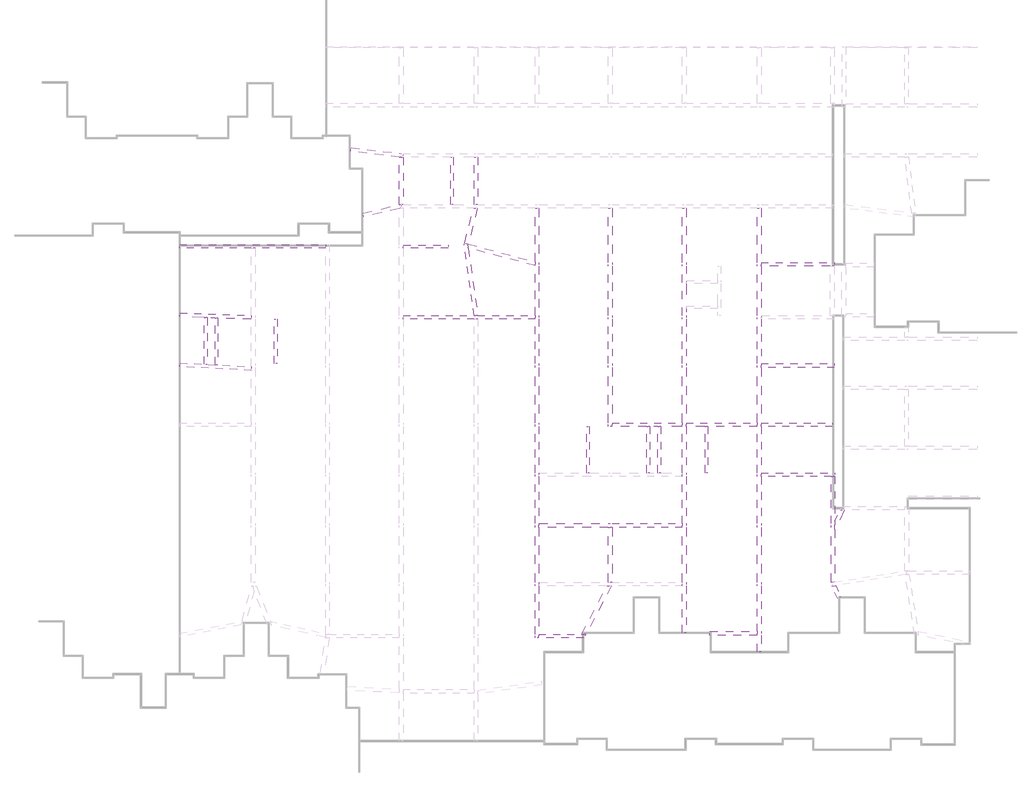
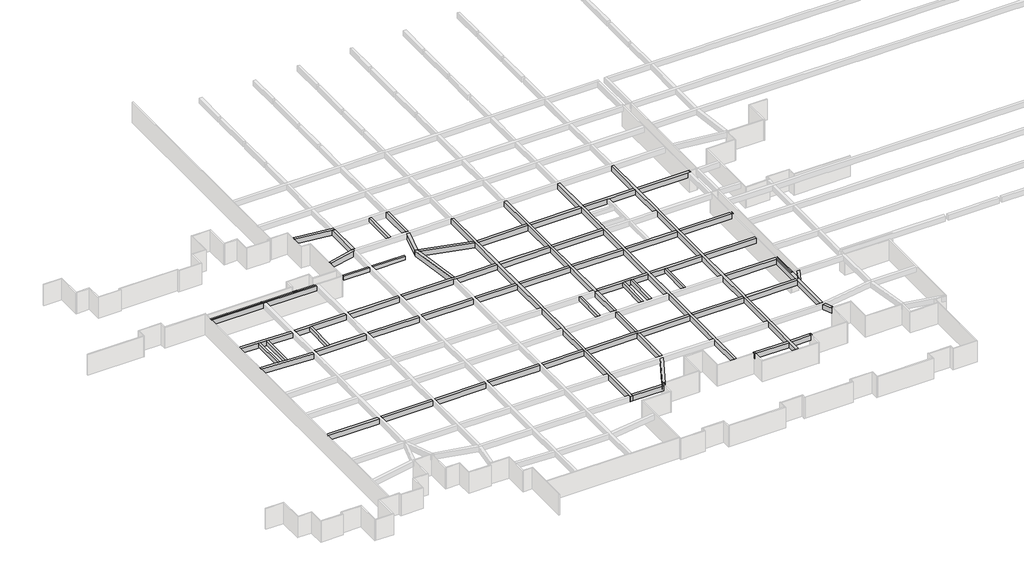
# One storey, part 10 of 16: 38 beams.
"""IFC4 building model written with IfcOpenShell, lengths in millimetres."""

from ifc_helpers import new_model, si_unit, frame, origin, place, context, project, spatial, polyline, outline, extrude, faceted_brep, element, save

model = new_model("IFC4")

# Units and contexts
model_context = context("Model", 3, world=origin())
ifc_project = project(units=[si_unit("LENGTHUNIT", "METRE", prefix="MILLI")], contexts=[model_context])

# Site, building, storey
site = spatial("IfcSite", under=ifc_project)
building = spatial("IfcBuilding", under=site)
storey = spatial("IfcBuildingStorey", under=building, Name="户型图", Elevation=0.0)

# Beams
placement = place(None, origin())
element("IfcBeam", 1, ObjectType="混凝土 - 矩形梁 : KL_beam", at=placement, inside=storey, context=model_context, shape_type="Brep", body=[
    faceted_brep([(202886.3957871, -166173.8814198, 3300.0), (202886.3957871, -166173.8814198, 2500.0), (202837.6480497, -166570.8998804, 2500.0), (202837.6480497, -166570.8998804, 3300.0), (208472.2780151, -167262.7454466, 3300.0), (208474.7427196, -167242.6720388, 3300.0), (208521.0257524, -166865.7269859, 3300.0), (208121.0257524, -166816.6131615, 3300.0), (208121.0257524, -167219.6170917, 3300.0), (208308.7932284, -167242.6720388, 3300.0), (208472.2780151, -167262.7454466, 2500.0), (208121.0257524, -167219.6170917, 2500.0), (208308.7932284, -167242.6720388, 2500.0), (208521.0257524, -166865.7269859, 2500.0), (208474.7427196, -167242.6720388, 2500.0), (208121.0257524, -166816.6131615, 2500.0)], [[[0, 1, 2, 3]], [[4, 5, 6, 7, 0, 3, 8, 9]], [[10, 4, 9, 8, 3, 2, 11, 12]], [[13, 14, 10, 12, 11, 2, 1, 15]], [[6, 13, 15, 1, 0, 7]], [[6, 5, 4, 10, 14, 13]]]),
])
element("IfcBeam", 2, ObjectType="混凝土 - 矩形梁 : KL_beam", at=placement, inside=storey, context=model_context, shape_type="Brep", body=[
    faceted_brep([(204160.2720993, -173284.8120655, 3300.0), (204160.2720993, -173284.8120655, 2500.0), (204250.2525211, -173674.5600915, 2500.0), (204250.2525211, -173674.5600915, 3300.0), (208320.403704, -172734.8916503, 3300.0), (208274.8294606, -172334.8916503, 3300.0), (208121.0257524, -172370.4000342, 3300.0), (208121.0257524, -172780.9216773, 3300.0), (208320.403704, -172734.8916503, 2500.0), (208121.0257524, -172780.9216773, 2500.0), (208274.8294606, -172334.8916503, 2500.0), (208121.0257524, -172370.4000342, 2500.0)], [[[0, 1, 2, 3]], [[4, 5, 6, 0, 3, 7]], [[8, 4, 7, 3, 2, 9]], [[10, 8, 9, 2, 1, 11]], [[5, 10, 11, 1, 0, 6]], [[5, 4, 8, 10]]]),
])
element("IfcBeam", 3, ObjectType="混凝土 - 矩形梁 : KL_beam", at=placement, inside=storey, context=model_context, shape_type="SweptSolid", body=[
    extrude(outline(polyline([(208308.7932284, -167242.6720388), (208472.2780151, -167262.7454466), (208474.7427196, -167242.6720388), (208521.0257524, -167242.6720388), (208521.0257524, -172334.8916503), (208274.8294606, -172334.8916503), (208121.0257524, -172370.4000342), (208121.0257524, -167242.6720388), (208308.7932284, -167242.6720388)])), frame((0.0, 0.0, 2500.0), z_axis=(0.0, 0.0, 1.0), x_axis=(1.0, 0.0, 0.0)), (0.0, 0.0, 1.0), 800.0),
])
element("IfcBeam", 4, ObjectType="混凝土 - 矩形梁 : KL_beam", at=placement, inside=storey, context=model_context, shape_type="SweptSolid", body=[
    extrude(outline(polyline([(216198.8904026, -167242.6720388), (216598.8904026, -167242.6720388), (216598.8904026, -172334.8916503), (216198.8904026, -172334.8916503), (216198.8904026, -167242.6720388)])), frame((0.0, 0.0, 2500.0), z_axis=(0.0, 0.0, 1.0), x_axis=(1.0, 0.0, 0.0)), (0.0, 0.0, 1.0), 800.0),
])
element("IfcBeam", 5, ObjectType="混凝土 - 矩形梁 : KL_beam", at=placement, inside=storey, context=model_context, shape_type="Brep", body=[
    faceted_brep([(215177.5544053, -176523.2702865, 3300.0), (215117.8929954, -176757.7149155, 3300.0), (216187.0478754, -184365.1471774, 3300.0), (216590.9789045, -184365.1471774, 3300.0), (215561.5342494, -177040.2678478, 3300.0), (215524.9612283, -176780.0372808, 3300.0), (215501.0573924, -176609.9526507, 3300.0), (216590.9789045, -184365.1471774, 2500.0), (215561.5342494, -177040.2678478, 2500.0), (215524.9612283, -176780.0372808, 2500.0), (215501.0573924, -176609.9526507, 2500.0), (215117.8929954, -176757.7149155, 2500.0), (215177.5544053, -176523.2702865, 2500.0), (216187.0478754, -184365.1471774, 2500.0)], [[[0, 1, 2, 3, 4, 5, 6]], [[6, 5, 4, 3, 7, 8, 9, 10]], [[11, 12, 10, 9, 8, 7, 13]], [[1, 11, 13, 2]], [[1, 0, 12, 11]], [[2, 13, 7, 3]], [[12, 0, 6, 10]]]),
])
element("IfcBeam", 6, ObjectType="混凝土 - 矩形梁 : KL_beam", at=placement, inside=storey, context=model_context, shape_type="Brep", body=[
    faceted_brep([(215501.0573924, -176609.9526507, 3300.0), (215524.9612283, -176780.0372808, 3300.0), (215563.9554515, -176626.8061348, 3300.0), (216554.3688646, -172734.8916503, 3300.0), (216141.6200419, -172734.8916503, 3300.0), (215177.5544053, -176523.2702865, 3300.0), (215524.9612283, -176780.0372808, 2500.0), (215563.9554515, -176626.8061348, 2500.0), (216554.3688646, -172734.8916503, 2500.0), (215501.0573924, -176609.9526507, 2500.0), (215177.5544053, -176523.2702865, 2500.0), (216141.6200419, -172734.8916503, 2500.0)], [[[0, 1, 2, 3, 4, 5]], [[1, 6, 7, 8, 3, 2]], [[6, 9, 10, 11, 8, 7]], [[10, 5, 4, 11]], [[1, 0, 9, 6]], [[4, 3, 8, 11]], [[9, 0, 5, 10]]]),
])
element("IfcBeam", 7, ObjectType="混凝土 - 矩形梁 : KL_beam", at=placement, inside=storey, context=model_context, shape_type="Brep", body=[
    faceted_brep([(222798.8904026, -219234.8916503, 3300.0), (223198.8904026, -219234.8916503, 3300.0), (223198.8904026, -218834.8916503, 3300.0), (223198.8904026, -213630.8034485, 3300.0), (223198.8904026, -213230.8034485, 3300.0), (223198.8904026, -207265.1471774, 3300.0), (223198.8904026, -206865.1471774, 3300.0), (223198.8904026, -201765.1471774, 3300.0), (223198.8904026, -201365.1471774, 3300.0), (223198.8904026, -196365.1471774, 3300.0), (223198.8904026, -195965.1471774, 3300.0), (223198.8904026, -189965.1471774, 3300.0), (223198.8904026, -189565.1471774, 3300.0), (223198.8904026, -184765.1471774, 3300.0), (223198.8904026, -184365.1471774, 3300.0), (223198.8904026, -179026.0461868, 3300.0), (223198.8904026, -178626.0461868, 3300.0), (223198.8904026, -172734.8916503, 3300.0), (222798.8904026, -172734.8916503, 3300.0), (222798.8904026, -178565.4011123, 3300.0), (222798.8904026, -178979.5115844, 3300.0), (222798.8904026, -184365.1471774, 3300.0), (222798.8904026, -184765.1471774, 3300.0), (222798.8904026, -189565.1471774, 3300.0), (222798.8904026, -189965.1471774, 3300.0), (222798.8904026, -195965.1471774, 3300.0), (222798.8904026, -196365.1471774, 3300.0), (222798.8904026, -201365.1471774, 3300.0), (222798.8904026, -201765.1471774, 3300.0), (222798.8904026, -206865.1471774, 3300.0), (222798.8904026, -207265.1471774, 3300.0), (222798.8904026, -213230.8034485, 3300.0), (222798.8904026, -213630.8034485, 3300.0), (222798.8904026, -218834.8916503, 3300.0), (222798.8904026, -219234.8916503, 2500.0), (222798.8904026, -172734.8916503, 2500.0), (222798.8904026, -178565.4011123, 2500.0), (222798.8904026, -178979.5115844, 2500.0), (222798.8904026, -184365.1471774, 2500.0), (222798.8904026, -184765.1471774, 2500.0), (222798.8904026, -189565.1471774, 2500.0), (222798.8904026, -189965.1471774, 2500.0), (222798.8904026, -195965.1471774, 2500.0), (222798.8904026, -196365.1471774, 2500.0), (222798.8904026, -201365.1471774, 2500.0), (222798.8904026, -201765.1471774, 2500.0), (222798.8904026, -206865.1471774, 2500.0), (222798.8904026, -207265.1471774, 2500.0), (222798.8904026, -213230.8034485, 2500.0), (222798.8904026, -213630.8034485, 2500.0), (222798.8904026, -218834.8916503, 2500.0), (223198.8904026, -219234.8916503, 2500.0), (223198.8904026, -172734.8916503, 2500.0), (223198.8904026, -178626.0461868, 2500.0), (223198.8904026, -179026.0461868, 2500.0), (223198.8904026, -184365.1471774, 2500.0), (223198.8904026, -184765.1471774, 2500.0), (223198.8904026, -189565.1471774, 2500.0), (223198.8904026, -189965.1471774, 2500.0), (223198.8904026, -195965.1471774, 2500.0), (223198.8904026, -196365.1471774, 2500.0), (223198.8904026, -201365.1471774, 2500.0), (223198.8904026, -201765.1471774, 2500.0), (223198.8904026, -206865.1471774, 2500.0), (223198.8904026, -207265.1471774, 2500.0), (223198.8904026, -213230.8034485, 2500.0), (223198.8904026, -213630.8034485, 2500.0), (223198.8904026, -218834.8916503, 2500.0)], [[[0, 1, 2, 3, 4, 5, 6, 7, 8, 9, 10, 11, 12, 13, 14, 15, 16, 17, 18, 19, 20, 21, 22, 23, 24, 25, 26, 27, 28, 29, 30, 31, 32, 33]], [[34, 0, 33, 32, 31, 30, 29, 28, 27, 26, 25, 24, 23, 22, 21, 20, 19, 18, 35, 36, 37, 38, 39, 40, 41, 42, 43, 44, 45, 46, 47, 48, 49, 50]], [[51, 34, 50, 49, 48, 47, 46, 45, 44, 43, 42, 41, 40, 39, 38, 37, 36, 35, 52, 53, 54, 55, 56, 57, 58, 59, 60, 61, 62, 63, 64, 65, 66, 67]], [[1, 51, 67, 66, 65, 64, 63, 62, 61, 60, 59, 58, 57, 56, 55, 54, 53, 52, 17, 16, 15, 14, 13, 12, 11, 10, 9, 8, 7, 6, 5, 4, 3, 2]], [[18, 17, 52, 35]], [[1, 0, 34, 51]]]),
])
element("IfcBeam", 8, ObjectType="混凝土 - 矩形梁 : KL_beam", at=placement, inside=storey, context=model_context, shape_type="Brep", body=[
    faceted_brep([(228058.8638251, -219234.8916503, 3300.0), (228271.5475977, -218834.8916503, 3300.0), (227818.5195775, -218834.8916503, 3300.0), (223198.8904026, -218834.8916503, 3300.0), (223198.8904026, -219234.8916503, 3300.0), (228058.8638251, -219234.8916503, 2500.0), (223198.8904026, -219234.8916503, 2500.0), (228271.5475977, -218834.8916503, 2500.0), (223198.8904026, -218834.8916503, 2500.0), (227818.5195775, -218834.8916503, 2500.0)], [[[0, 1, 2, 3, 4]], [[5, 0, 4, 6]], [[7, 5, 6, 8, 9]], [[1, 7, 9, 8, 3, 2]], [[4, 3, 8, 6]], [[1, 0, 5, 7]]]),
])
element("IfcBeam", 9, ObjectType="混凝土 - 矩形梁 : KL_beam", at=placement, inside=storey, context=model_context, shape_type="Brep", body=[
    faceted_brep([(230718.438254, -196365.1471774, 3300.0), (231118.438254, -196365.1471774, 3300.0), (231118.438254, -195965.1471774, 3300.0), (231118.438254, -189965.1471774, 3300.0), (231118.438254, -189565.1471774, 3300.0), (231118.438254, -184765.1471774, 3300.0), (231118.438254, -184365.1471774, 3300.0), (231118.438254, -179026.0461868, 3300.0), (231118.438254, -178626.0461868, 3300.0), (231118.438254, -172734.8916503, 3300.0), (230718.438254, -172734.8916503, 3300.0), (230718.438254, -178626.0461868, 3300.0), (230718.438254, -179026.0461868, 3300.0), (230718.438254, -184365.1471774, 3300.0), (230718.438254, -184765.1471774, 3300.0), (230718.438254, -189565.1471774, 3300.0), (230718.438254, -189965.1471774, 3300.0), (230718.438254, -195965.1471774, 3300.0), (230718.438254, -196365.1471774, 2500.0), (230718.438254, -172734.8916503, 2500.0), (230718.438254, -178626.0461868, 2500.0), (230718.438254, -179026.0461868, 2500.0), (230718.438254, -184365.1471774, 2500.0), (230718.438254, -184765.1471774, 2500.0), (230718.438254, -189565.1471774, 2500.0), (230718.438254, -189965.1471774, 2500.0), (230718.438254, -195965.1471774, 2500.0), (231118.438254, -196365.1471774, 2500.0), (231118.438254, -172734.8916503, 2500.0), (231118.438254, -178626.0461868, 2500.0), (231118.438254, -179026.0461868, 2500.0), (231118.438254, -184365.1471774, 2500.0), (231118.438254, -184765.1471774, 2500.0), (231118.438254, -189565.1471774, 2500.0), (231118.438254, -189965.1471774, 2500.0), (231118.438254, -195965.1471774, 2500.0)], [[[0, 1, 2, 3, 4, 5, 6, 7, 8, 9, 10, 11, 12, 13, 14, 15, 16, 17]], [[18, 0, 17, 16, 15, 14, 13, 12, 11, 10, 19, 20, 21, 22, 23, 24, 25, 26]], [[27, 18, 26, 25, 24, 23, 22, 21, 20, 19, 28, 29, 30, 31, 32, 33, 34, 35]], [[1, 27, 35, 34, 33, 32, 31, 30, 29, 28, 9, 8, 7, 6, 5, 4, 3, 2]], [[10, 9, 28, 19]], [[1, 0, 18, 27]]]),
])
element("IfcBeam", 10, ObjectType="混凝土 - 矩形梁 : KL_beam", at=placement, inside=storey, context=model_context, shape_type="Brep", body=[
    faceted_brep([(239118.438254, -218673.2637363, 3300.0), (238718.438254, -218673.2637363, 3300.0), (238718.438254, -218673.2637363, 2500.0), (239118.438254, -218673.2637363, 2500.0), (239118.438254, -213630.8034485, 3300.0), (239118.438254, -213230.8034485, 3300.0), (239118.438254, -207265.1471774, 3300.0), (239118.438254, -206865.1471774, 3300.0), (239118.438254, -201765.1471774, 3300.0), (239118.438254, -201365.1471774, 3300.0), (239118.438254, -196365.1471774, 3300.0), (239118.438254, -195965.1471774, 3300.0), (239118.438254, -189965.1471774, 3300.0), (239118.438254, -189565.1471774, 3300.0), (239118.438254, -184765.1471774, 3300.0), (239118.438254, -184365.1471774, 3300.0), (239118.438254, -183615.1471774, 3300.0), (239118.438254, -183315.1471774, 3300.0), (239118.438254, -180876.0461868, 3300.0), (239118.438254, -180576.0461868, 3300.0), (239118.438254, -179026.0461868, 3300.0), (239118.438254, -178626.0461868, 3300.0), (239118.438254, -172734.8916503, 3300.0), (238718.438254, -172734.8916503, 3300.0), (238718.438254, -178626.0461868, 3300.0), (238718.438254, -179026.0461868, 3300.0), (238718.438254, -184365.1471774, 3300.0), (238718.438254, -184765.1471774, 3300.0), (238718.438254, -189565.1471774, 3300.0), (238718.438254, -189965.1471774, 3300.0), (238718.438254, -195965.1471774, 3300.0), (238718.438254, -196365.1471774, 3300.0), (238718.438254, -201365.1471774, 3300.0), (238718.438254, -201765.1471774, 3300.0), (238718.438254, -206865.1471774, 3300.0), (238718.438254, -207265.1471774, 3300.0), (238718.438254, -213230.8034485, 3300.0), (238718.438254, -213630.8034485, 3300.0), (238718.438254, -172734.8916503, 2500.0), (238718.438254, -178626.0461868, 2500.0), (238718.438254, -179026.0461868, 2500.0), (238718.438254, -184365.1471774, 2500.0), (238718.438254, -184765.1471774, 2500.0), (238718.438254, -189565.1471774, 2500.0), (238718.438254, -189965.1471774, 2500.0), (238718.438254, -195965.1471774, 2500.0), (238718.438254, -196365.1471774, 2500.0), (238718.438254, -201365.1471774, 2500.0), (238718.438254, -201765.1471774, 2500.0), (238718.438254, -206865.1471774, 2500.0), (238718.438254, -207265.1471774, 2500.0), (238718.438254, -213230.8034485, 2500.0), (238718.438254, -213630.8034485, 2500.0), (239118.438254, -172734.8916503, 2500.0), (239118.438254, -178626.0461868, 2500.0), (239118.438254, -179026.0461868, 2500.0), (239118.438254, -184365.1471774, 2500.0), (239118.438254, -184765.1471774, 2500.0), (239118.438254, -189565.1471774, 2500.0), (239118.438254, -189965.1471774, 2500.0), (239118.438254, -195965.1471774, 2500.0), (239118.438254, -196365.1471774, 2500.0), (239118.438254, -201365.1471774, 2500.0), (239118.438254, -201765.1471774, 2500.0), (239118.438254, -206865.1471774, 2500.0), (239118.438254, -207265.1471774, 2500.0), (239118.438254, -213230.8034485, 2500.0), (239118.438254, -213630.8034485, 2500.0)], [[[0, 1, 2, 3]], [[1, 0, 4, 5, 6, 7, 8, 9, 10, 11, 12, 13, 14, 15, 16, 17, 18, 19, 20, 21, 22, 23, 24, 25, 26, 27, 28, 29, 30, 31, 32, 33, 34, 35, 36, 37]], [[2, 1, 37, 36, 35, 34, 33, 32, 31, 30, 29, 28, 27, 26, 25, 24, 23, 38, 39, 40, 41, 42, 43, 44, 45, 46, 47, 48, 49, 50, 51, 52]], [[3, 2, 52, 51, 50, 49, 48, 47, 46, 45, 44, 43, 42, 41, 40, 39, 38, 53, 54, 55, 56, 57, 58, 59, 60, 61, 62, 63, 64, 65, 66, 67]], [[0, 3, 67, 66, 65, 64, 63, 62, 61, 60, 59, 58, 57, 56, 55, 54, 53, 22, 21, 20, 19, 18, 17, 16, 15, 14, 13, 12, 11, 10, 9, 8, 7, 6, 5, 4]], [[23, 22, 53, 38]]]),
])
element("IfcBeam", 11, ObjectType="混凝土 - 矩形梁 : KL_beam", at=placement, inside=storey, context=model_context, shape_type="Brep", body=[
    faceted_brep([(247218.438254, -220773.3230967, 3300.0), (246818.438254, -220773.3230967, 3300.0), (246818.438254, -220773.3230967, 2500.0), (247218.438254, -220773.3230967, 2500.0), (247218.438254, -218948.6524453, 3300.0), (247218.438254, -218548.6524453, 3300.0), (247218.438254, -213630.8034485, 3300.0), (247218.438254, -213230.8034485, 3300.0), (247218.438254, -207265.1471774, 3300.0), (247218.438254, -206865.1471774, 3300.0), (247218.438254, -201765.1471774, 3300.0), (247218.438254, -201365.1471774, 3300.0), (247218.438254, -196365.1471774, 3300.0), (247218.438254, -195965.1471774, 3300.0), (247218.438254, -189965.1471774, 3300.0), (247218.438254, -189565.1471774, 3300.0), (247218.438254, -184765.1471774, 3300.0), (247218.438254, -184365.1471774, 3300.0), (247218.438254, -179026.0461868, 3300.0), (247218.438254, -178626.0461868, 3300.0), (247218.438254, -172734.8916503, 3300.0), (246818.438254, -172734.8916503, 3300.0), (246818.438254, -178626.0461868, 3300.0), (246818.438254, -179026.0461868, 3300.0), (246818.438254, -184365.1471774, 3300.0), (246818.438254, -184765.1471774, 3300.0), (246818.438254, -189565.1471774, 3300.0), (246818.438254, -189965.1471774, 3300.0), (246818.438254, -195965.1471774, 3300.0), (246818.438254, -196365.1471774, 3300.0), (246818.438254, -201365.1471774, 3300.0), (246818.438254, -201765.1471774, 3300.0), (246818.438254, -206865.1471774, 3300.0), (246818.438254, -207265.1471774, 3300.0), (246818.438254, -213230.8034485, 3300.0), (246818.438254, -213630.8034485, 3300.0), (246818.438254, -218548.6524453, 3300.0), (246818.438254, -218948.6524453, 3300.0), (246818.438254, -172734.8916503, 2500.0), (246818.438254, -178626.0461868, 2500.0), (246818.438254, -179026.0461868, 2500.0), (246818.438254, -184365.1471774, 2500.0), (246818.438254, -184765.1471774, 2500.0), (246818.438254, -189565.1471774, 2500.0), (246818.438254, -189965.1471774, 2500.0), (246818.438254, -195965.1471774, 2500.0), (246818.438254, -196365.1471774, 2500.0), (246818.438254, -201365.1471774, 2500.0), (246818.438254, -201765.1471774, 2500.0), (246818.438254, -206865.1471774, 2500.0), (246818.438254, -207265.1471774, 2500.0), (246818.438254, -213230.8034485, 2500.0), (246818.438254, -213630.8034485, 2500.0), (246818.438254, -218548.6524453, 2500.0), (246818.438254, -218948.6524453, 2500.0), (247218.438254, -172734.8916503, 2500.0), (247218.438254, -178626.0461868, 2500.0), (247218.438254, -179026.0461868, 2500.0), (247218.438254, -184365.1471774, 2500.0), (247218.438254, -184765.1471774, 2500.0), (247218.438254, -189565.1471774, 2500.0), (247218.438254, -189965.1471774, 2500.0), (247218.438254, -195965.1471774, 2500.0), (247218.438254, -196365.1471774, 2500.0), (247218.438254, -201365.1471774, 2500.0), (247218.438254, -201765.1471774, 2500.0), (247218.438254, -206865.1471774, 2500.0), (247218.438254, -207265.1471774, 2500.0), (247218.438254, -213230.8034485, 2500.0), (247218.438254, -213630.8034485, 2500.0), (247218.438254, -218548.6524453, 2500.0), (247218.438254, -218948.6524453, 2500.0)], [[[0, 1, 2, 3]], [[1, 0, 4, 5, 6, 7, 8, 9, 10, 11, 12, 13, 14, 15, 16, 17, 18, 19, 20, 21, 22, 23, 24, 25, 26, 27, 28, 29, 30, 31, 32, 33, 34, 35, 36, 37]], [[2, 1, 37, 36, 35, 34, 33, 32, 31, 30, 29, 28, 27, 26, 25, 24, 23, 22, 21, 38, 39, 40, 41, 42, 43, 44, 45, 46, 47, 48, 49, 50, 51, 52, 53, 54]], [[3, 2, 54, 53, 52, 51, 50, 49, 48, 47, 46, 45, 44, 43, 42, 41, 40, 39, 38, 55, 56, 57, 58, 59, 60, 61, 62, 63, 64, 65, 66, 67, 68, 69, 70, 71]], [[0, 3, 71, 70, 69, 68, 67, 66, 65, 64, 63, 62, 61, 60, 59, 58, 57, 56, 55, 20, 19, 18, 17, 16, 15, 14, 13, 12, 11, 10, 9, 8, 7, 6, 5, 4]], [[21, 20, 55, 38]]]),
])
element("IfcBeam", 12, ObjectType="混凝土 - 矩形梁 : KL_beam", at=placement, inside=storey, context=model_context, shape_type="Brep", body=[
    faceted_brep([(192508.6297316, -184365.1471774, 3300.0), (192508.6297316, -184765.1471774, 3300.0), (194594.1756261, -184765.1471774, 3300.0), (194894.1756261, -184765.1471774, 3300.0), (200145.9052003, -184765.1471774, 3300.0), (200145.9052003, -184365.1471774, 3300.0), (192508.6297316, -184765.1471774, 2500.0), (200145.9052003, -184765.1471774, 2500.0), (192508.6297316, -184365.1471774, 2500.0), (200145.9052003, -184365.1471774, 2500.0)], [[[0, 1, 2, 3, 4, 5]], [[1, 6, 7, 4, 3, 2]], [[6, 8, 9, 7]], [[8, 0, 5, 9]], [[1, 0, 8, 6]], [[5, 4, 7, 9]]]),
    faceted_brep([(238718.438254, -184365.1471774, 3300.0), (238718.438254, -184765.1471774, 3300.0), (238718.438254, -184765.1471774, 2500.0), (238718.438254, -184365.1471774, 2500.0), (231118.438254, -184765.1471774, 3300.0), (231118.438254, -184365.1471774, 3300.0), (231118.438254, -184365.1471774, 2500.0), (231118.438254, -184765.1471774, 2500.0)], [[[0, 1, 2, 3]], [[4, 5, 6, 7]], [[1, 0, 5, 4]], [[2, 1, 4, 7]], [[3, 2, 7, 6]], [[0, 3, 6, 5]]]),
    faceted_brep([(208121.0257524, -184365.1471774, 3300.0), (208121.0257524, -184765.1471774, 3300.0), (208121.0257524, -184765.1471774, 2500.0), (208121.0257524, -184365.1471774, 2500.0), (200545.9052003, -184765.1471774, 3300.0), (200545.9052003, -184365.1471774, 3300.0), (200545.9052003, -184365.1471774, 2500.0), (200545.9052003, -184765.1471774, 2500.0)], [[[0, 1, 2, 3]], [[4, 5, 6, 7]], [[1, 0, 5, 4]], [[2, 1, 4, 7]], [[3, 2, 7, 6]], [[0, 3, 6, 5]]]),
    faceted_brep([(208521.0257524, -184765.1471774, 3300.0), (208521.0257524, -184365.1471774, 3300.0), (208521.0257524, -184365.1471774, 2500.0), (208521.0257524, -184765.1471774, 2500.0), (222798.8904026, -184365.1471774, 3300.0), (222798.8904026, -184765.1471774, 3300.0), (222798.8904026, -184765.1471774, 2500.0), (222798.8904026, -184365.1471774, 2500.0), (216206.9772993, -184765.1471774, 3300.0), (216606.9772993, -184765.1471774, 3300.0), (216590.9789045, -184365.1471774, 3300.0), (216187.0478754, -184365.1471774, 3300.0), (216206.9772993, -184765.1471774, 2500.0), (216606.9772993, -184765.1471774, 2500.0), (216187.0478754, -184365.1471774, 2500.0), (216590.9789045, -184365.1471774, 2500.0)], [[[0, 1, 2, 3]], [[4, 5, 6, 7]], [[1, 0, 8, 9, 5, 4, 10, 11]], [[0, 3, 12, 13, 6, 5, 9, 8]], [[3, 2, 14, 15, 7, 6, 13, 12]], [[2, 1, 11, 10, 4, 7, 15, 14]]]),
    faceted_brep([(223198.8904026, -184365.1471774, 3300.0), (223198.8904026, -184765.1471774, 3300.0), (230718.438254, -184765.1471774, 3300.0), (230718.438254, -184365.1471774, 3300.0), (223198.8904026, -184765.1471774, 2500.0), (230718.438254, -184765.1471774, 2500.0), (223198.8904026, -184365.1471774, 2500.0), (230718.438254, -184365.1471774, 2500.0)], [[[0, 1, 2, 3]], [[1, 4, 5, 2]], [[4, 6, 7, 5]], [[6, 0, 3, 7]], [[1, 0, 6, 4]], [[3, 2, 5, 7]]]),
])
element("IfcBeam", 13, ObjectType="混凝土 - 矩形梁 : KL_beam", at=placement, inside=storey, context=model_context, shape_type="SweptSolid", body=[
    extrude(outline(polyline([(215561.5342494, -177040.2678478), (215524.9612283, -176780.0372808), (215563.9554515, -176626.8061348), (222798.8904026, -178565.4011123), (222798.8904026, -178979.5115844), (215561.5342494, -177040.2678478)])), frame((0.0, 0.0, 2500.0), z_axis=(0.0, 0.0, 1.0), x_axis=(1.0, 0.0, 0.0)), (0.0, 0.0, 1.0), 800.0),
])
element("IfcBeam", 14, ObjectType="混凝土 - 矩形梁 : KL_beam", at=placement, inside=storey, context=model_context, shape_type="Brep", body=[
    faceted_brep([(223198.8904026, -178626.0461868, 3300.0), (223198.8904026, -179026.0461868, 3300.0), (230718.438254, -179026.0461868, 3300.0), (230718.438254, -178626.0461868, 3300.0), (223198.8904026, -179026.0461868, 2500.0), (230718.438254, -179026.0461868, 2500.0), (223198.8904026, -178626.0461868, 2500.0), (230718.438254, -178626.0461868, 2500.0)], [[[0, 1, 2, 3]], [[1, 4, 5, 2]], [[4, 6, 7, 5]], [[6, 0, 3, 7]], [[1, 0, 6, 4]], [[3, 2, 5, 7]]]),
    faceted_brep([(231118.438254, -179026.0461868, 3300.0), (231118.438254, -178626.0461868, 3300.0), (231118.438254, -178626.0461868, 2500.0), (231118.438254, -179026.0461868, 2500.0), (238718.438254, -178626.0461868, 3300.0), (238718.438254, -179026.0461868, 3300.0), (238718.438254, -179026.0461868, 2500.0), (238718.438254, -178626.0461868, 2500.0)], [[[0, 1, 2, 3]], [[4, 5, 6, 7]], [[1, 0, 5, 4]], [[0, 3, 6, 5]], [[3, 2, 7, 6]], [[2, 1, 4, 7]]]),
    faceted_brep([(239118.438254, -178626.0461868, 3300.0), (239118.438254, -179026.0461868, 3300.0), (242568.438254, -179026.0461868, 3300.0), (242868.438254, -179026.0461868, 3300.0), (246818.438254, -179026.0461868, 3300.0), (246818.438254, -178626.0461868, 3300.0), (239118.438254, -179026.0461868, 2500.0), (246818.438254, -179026.0461868, 2500.0), (239118.438254, -178626.0461868, 2500.0), (246818.438254, -178626.0461868, 2500.0)], [[[0, 1, 2, 3, 4, 5]], [[1, 6, 7, 4, 3, 2]], [[6, 8, 9, 7]], [[8, 0, 5, 9]], [[1, 0, 8, 6]], [[5, 4, 7, 9]]]),
    faceted_brep([(247218.438254, -179026.0461868, 3300.0), (247218.438254, -178626.0461868, 3300.0), (247218.438254, -178626.0461868, 2500.0), (247218.438254, -179026.0461868, 2500.0), (255118.438254, -178626.0461868, 3300.0), (255118.438254, -179026.0461868, 3300.0), (255118.438254, -179026.0461868, 2500.0), (255118.438254, -178626.0461868, 2500.0), (254718.438254, -179026.0461868, 3300.0), (254718.438254, -179026.0461868, 2500.0)], [[[0, 1, 2, 3]], [[4, 5, 6, 7]], [[5, 4, 1, 0, 8]], [[6, 5, 8, 0, 3, 9]], [[7, 6, 9, 3, 2]], [[4, 7, 2, 1]]]),
])
element("IfcBeam", 15, ObjectType="混凝土 - 矩形梁 : KL_beam", at=placement, inside=storey, context=model_context, shape_type="Brep", body=[
    faceted_brep([(184345.9052003, -177080.869332, 3300.0), (184345.9052003, -176680.869332, 3300.0), (184345.9052003, -176680.869332, 2500.0), (184345.9052003, -177080.869332, 2500.0), (192108.6297316, -177080.869332, 3300.0), (192508.6297316, -177080.869332, 3300.0), (200145.9052003, -177080.869332, 3300.0), (200145.9052003, -176680.869332, 3300.0), (200145.9052003, -176680.869332, 2500.0), (200145.9052003, -177080.869332, 2500.0), (192508.6297316, -177080.869332, 2500.0), (192108.6297316, -177080.869332, 2500.0)], [[[0, 1, 2, 3]], [[1, 0, 4, 5, 6, 7]], [[2, 1, 7, 8]], [[3, 2, 8, 9, 10, 11]], [[0, 3, 11, 10, 9, 6, 5, 4]], [[7, 6, 9, 8]]]),
])
element("IfcBeam", 16, ObjectType="混凝土 - 矩形梁 : KL_beam", at=placement, inside=storey, context=model_context, shape_type="Brep", body=[
    faceted_brep([(184367.3625426, -184487.9539253, 3300.0), (184381.3223413, -184088.1975945, 3300.0), (184381.3223413, -184088.1975945, 2500.0), (184367.3625426, -184487.9539253, 2500.0), (187022.6367576, -184580.6781441, 3300.0), (187322.6367576, -184591.154375, 3300.0), (188191.4243298, -184621.4931055, 3300.0), (188491.4243298, -184631.9693364, 3300.0), (192108.6297316, -184758.2849324, 3300.0), (192108.6297316, -184358.0411147, 3300.0), (192108.6297316, -184358.0411147, 2500.0), (192108.6297316, -184758.2849324, 2500.0)], [[[0, 1, 2, 3]], [[1, 0, 4, 5, 6, 7, 8, 9]], [[2, 1, 9, 10]], [[3, 2, 10, 11]], [[0, 3, 11, 8, 7, 6, 5, 4]], [[9, 8, 11, 10]]]),
])
element("IfcBeam", 17, ObjectType="混凝土 - 矩形梁 : KL_beam", at=placement, inside=storey, context=model_context, shape_type="Brep", body=[
    faceted_brep([(184363.9013118, -189889.0560732, 3300.0), (184384.8356943, -189489.6042592, 3300.0), (184384.8356943, -189489.6042592, 2500.0), (184363.9013118, -189889.0560732, 2500.0), (192108.6297316, -190294.9400908, 3300.0), (192108.6297316, -189894.3911524, 3300.0), (188491.4243298, -189704.8214501, 3300.0), (188191.4243298, -189689.0991163, 3300.0), (187322.6367576, -189643.567889, 3300.0), (187022.6367576, -189627.8455552, 3300.0), (192108.6297316, -189894.3911524, 2500.0), (192108.6297316, -190294.9400908, 2500.0)], [[[0, 1, 2, 3]], [[1, 0, 4, 5, 6, 7, 8, 9]], [[2, 1, 9, 8, 7, 6, 5, 10]], [[3, 2, 10, 11]], [[0, 3, 11, 4]], [[5, 4, 11, 10]]]),
])
element("IfcBeam", 18, ObjectType="混凝土 - 矩形梁 : KL_beam", at=placement, inside=storey, context=model_context, shape_type="Brep", body=[
    faceted_brep([(231118.438254, -195965.1471774, 3300.0), (231118.438254, -196365.1471774, 3300.0), (234868.438254, -196365.1471774, 3300.0), (235168.438254, -196365.1471774, 3300.0), (236068.438254, -196365.1471774, 3300.0), (236368.438254, -196365.1471774, 3300.0), (238718.438254, -196365.1471774, 3300.0), (238718.438254, -195965.1471774, 3300.0), (231118.438254, -196365.1471774, 2500.0), (238718.438254, -196365.1471774, 2500.0), (231118.438254, -195965.1471774, 2500.0), (238718.438254, -195965.1471774, 2500.0)], [[[0, 1, 2, 3, 4, 5, 6, 7]], [[1, 8, 9, 6, 5, 4, 3, 2]], [[8, 10, 11, 9]], [[10, 0, 7, 11]], [[1, 0, 10, 8]], [[7, 6, 9, 11]]]),
])
element("IfcBeam", 19, ObjectType="混凝土 - 矩形梁 : KL_beam", at=placement, inside=storey, context=model_context, shape_type="Brep", body=[
    faceted_brep([(239118.438254, -195965.1471774, 3300.0), (239118.438254, -196365.1471774, 3300.0), (241168.438254, -196365.1471774, 3300.0), (241468.438254, -196365.1471774, 3300.0), (246818.438254, -196365.1471774, 3300.0), (246818.438254, -195965.1471774, 3300.0), (239118.438254, -196365.1471774, 2500.0), (246818.438254, -196365.1471774, 2500.0), (239118.438254, -195965.1471774, 2500.0), (246818.438254, -195965.1471774, 2500.0)], [[[0, 1, 2, 3, 4, 5]], [[1, 6, 7, 4, 3, 2]], [[6, 8, 9, 7]], [[8, 0, 5, 9]], [[1, 0, 8, 6]], [[5, 4, 7, 9]]]),
])
element("IfcBeam", 20, ObjectType="混凝土 - 矩形梁 : KL_beam", at=placement, inside=storey, context=model_context, shape_type="Brep", body=[
    faceted_brep([(255153.6937038, -189565.1471774, 3300.0), (255153.6937038, -189965.1471774, 3300.0), (255153.6937038, -189965.1471774, 2500.0), (255153.6937038, -189565.1471774, 2500.0), (247218.438254, -189565.1471774, 3300.0), (247218.438254, -189965.1471774, 3300.0), (247218.438254, -189965.1471774, 2500.0), (247218.438254, -189565.1471774, 2500.0)], [[[0, 1, 2, 3]], [[1, 0, 4, 5]], [[2, 1, 5, 6]], [[3, 2, 6, 7]], [[0, 3, 7, 4]], [[5, 4, 7, 6]]]),
    faceted_brep([(192508.6297316, -189965.1471774, 3300.0), (192508.6297316, -189565.1471774, 3300.0), (192508.6297316, -189565.1471774, 2500.0), (192508.6297316, -189965.1471774, 2500.0), (200145.9052003, -189565.1471774, 3300.0), (200145.9052003, -189965.1471774, 3300.0), (200145.9052003, -189965.1471774, 2500.0), (200145.9052003, -189565.1471774, 2500.0), (194894.1756261, -189565.1471774, 3300.0), (194594.1756261, -189565.1471774, 3300.0)], [[[0, 1, 2, 3]], [[4, 5, 6, 7]], [[1, 0, 5, 4, 8, 9]], [[0, 3, 6, 5]], [[3, 2, 7, 6]], [[2, 1, 9, 8, 4, 7]]]),
    faceted_brep([(208121.0257524, -189565.1471774, 3300.0), (208121.0257524, -189965.1471774, 3300.0), (208121.0257524, -189965.1471774, 2500.0), (208121.0257524, -189565.1471774, 2500.0), (200545.9052003, -189565.1471774, 3300.0), (200545.9052003, -189965.1471774, 3300.0), (200545.9052003, -189965.1471774, 2500.0), (200545.9052003, -189565.1471774, 2500.0)], [[[0, 1, 2, 3]], [[1, 0, 4, 5]], [[2, 1, 5, 6]], [[3, 2, 6, 7]], [[0, 3, 7, 4]], [[5, 4, 7, 6]]]),
    faceted_brep([(208521.0257524, -189965.1471774, 3300.0), (208521.0257524, -189565.1471774, 3300.0), (208521.0257524, -189565.1471774, 2500.0), (208521.0257524, -189965.1471774, 2500.0), (216206.9772993, -189565.1471774, 3300.0), (216206.9772993, -189965.1471774, 3300.0), (216206.9772993, -189965.1471774, 2500.0), (216206.9772993, -189565.1471774, 2500.0)], [[[0, 1, 2, 3]], [[4, 5, 6, 7]], [[1, 0, 5, 4]], [[0, 3, 6, 5]], [[3, 2, 7, 6]], [[2, 1, 4, 7]]]),
    faceted_brep([(216606.9772993, -189965.1471774, 3300.0), (216606.9772993, -189565.1471774, 3300.0), (216606.9772993, -189565.1471774, 2500.0), (216606.9772993, -189965.1471774, 2500.0), (222798.8904026, -189565.1471774, 3300.0), (222798.8904026, -189965.1471774, 3300.0), (222798.8904026, -189965.1471774, 2500.0), (222798.8904026, -189565.1471774, 2500.0)], [[[0, 1, 2, 3]], [[4, 5, 6, 7]], [[1, 0, 5, 4]], [[0, 3, 6, 5]], [[3, 2, 7, 6]], [[2, 1, 4, 7]]]),
    faceted_brep([(223198.8904026, -189965.1471774, 3300.0), (223198.8904026, -189565.1471774, 3300.0), (223198.8904026, -189565.1471774, 2500.0), (223198.8904026, -189965.1471774, 2500.0), (230718.438254, -189565.1471774, 3300.0), (230718.438254, -189965.1471774, 3300.0), (230718.438254, -189965.1471774, 2500.0), (230718.438254, -189565.1471774, 2500.0)], [[[0, 1, 2, 3]], [[4, 5, 6, 7]], [[1, 0, 5, 4]], [[0, 3, 6, 5]], [[3, 2, 7, 6]], [[2, 1, 4, 7]]]),
    faceted_brep([(231118.438254, -189965.1471774, 3300.0), (231118.438254, -189565.1471774, 3300.0), (231118.438254, -189565.1471774, 2500.0), (231118.438254, -189965.1471774, 2500.0), (238718.438254, -189565.1471774, 3300.0), (238718.438254, -189965.1471774, 3300.0), (238718.438254, -189965.1471774, 2500.0), (238718.438254, -189565.1471774, 2500.0)], [[[0, 1, 2, 3]], [[4, 5, 6, 7]], [[1, 0, 5, 4]], [[0, 3, 6, 5]], [[3, 2, 7, 6]], [[2, 1, 4, 7]]]),
    faceted_brep([(239118.438254, -189965.1471774, 3300.0), (239118.438254, -189565.1471774, 3300.0), (239118.438254, -189565.1471774, 2500.0), (239118.438254, -189965.1471774, 2500.0), (246818.438254, -189565.1471774, 3300.0), (246818.438254, -189965.1471774, 3300.0), (246818.438254, -189965.1471774, 2500.0), (246818.438254, -189565.1471774, 2500.0), (242868.438254, -189565.1471774, 3300.0), (242568.438254, -189565.1471774, 3300.0)], [[[0, 1, 2, 3]], [[4, 5, 6, 7]], [[1, 0, 5, 4, 8, 9]], [[0, 3, 6, 5]], [[3, 2, 7, 6]], [[2, 1, 9, 8, 4, 7]]]),
])
element("IfcBeam", 21, ObjectType="混凝土 - 矩形梁 : KL_beam", at=placement, inside=storey, context=model_context, shape_type="Brep", body=[
    faceted_brep([(184374.3285911, -206865.1471774, 3300.0), (184374.3285911, -206865.1471774, 2500.0), (184374.3285911, -207265.1471774, 2500.0), (184374.3285911, -207265.1471774, 3300.0), (192108.6297316, -206865.1471774, 3300.0), (192108.6297316, -207265.1471774, 3300.0), (192108.6297316, -207265.1471774, 2500.0), (192108.6297316, -206865.1471774, 2500.0)], [[[0, 1, 2, 3]], [[4, 5, 6, 7]], [[0, 3, 5, 4]], [[3, 2, 6, 5]], [[2, 1, 7, 6]], [[1, 0, 4, 7]]]),
    faceted_brep([(208521.0257524, -206865.1471774, 3300.0), (208521.0257524, -207265.1471774, 3300.0), (216206.9772993, -207265.1471774, 3300.0), (216206.9772993, -206865.1471774, 3300.0), (208521.0257524, -207265.1471774, 2500.0), (216206.9772993, -207265.1471774, 2500.0), (208521.0257524, -206865.1471774, 2500.0), (216206.9772993, -206865.1471774, 2500.0)], [[[0, 1, 2, 3]], [[1, 4, 5, 2]], [[4, 6, 7, 5]], [[6, 0, 3, 7]], [[1, 0, 6, 4]], [[3, 2, 5, 7]]]),
    faceted_brep([(208121.0257524, -206865.1471774, 3300.0), (208121.0257524, -207265.1471774, 3300.0), (208121.0257524, -207265.1471774, 2500.0), (208121.0257524, -206865.1471774, 2500.0), (200545.9052003, -206865.1471774, 3300.0), (200545.9052003, -207265.1471774, 3300.0), (200545.9052003, -207265.1471774, 2500.0), (200545.9052003, -206865.1471774, 2500.0)], [[[0, 1, 2, 3]], [[1, 0, 4, 5]], [[2, 1, 5, 6]], [[3, 2, 6, 7]], [[0, 3, 7, 4]], [[5, 4, 7, 6]]]),
    faceted_brep([(216606.9772993, -207265.1471774, 3300.0), (216606.9772993, -206865.1471774, 3300.0), (216606.9772993, -206865.1471774, 2500.0), (216606.9772993, -207265.1471774, 2500.0), (222798.8904026, -206865.1471774, 3300.0), (222798.8904026, -207265.1471774, 3300.0), (222798.8904026, -207265.1471774, 2500.0), (222798.8904026, -206865.1471774, 2500.0)], [[[0, 1, 2, 3]], [[4, 5, 6, 7]], [[1, 0, 5, 4]], [[0, 3, 6, 5]], [[3, 2, 7, 6]], [[2, 1, 4, 7]]]),
    faceted_brep([(223198.8904026, -206865.1471774, 3300.0), (223198.8904026, -207265.1471774, 3300.0), (230718.438254, -207265.1471774, 3300.0), (231118.438254, -207265.1471774, 3300.0), (238718.438254, -207265.1471774, 3300.0), (238718.438254, -206865.1471774, 3300.0), (231118.438254, -206865.1471774, 3300.0), (230718.438254, -206865.1471774, 3300.0), (223198.8904026, -207265.1471774, 2500.0), (230718.438254, -207265.1471774, 2500.0), (231118.438254, -207265.1471774, 2500.0), (238718.438254, -207265.1471774, 2500.0), (223198.8904026, -206865.1471774, 2500.0), (230718.438254, -206865.1471774, 2500.0), (231118.438254, -206865.1471774, 2500.0), (238718.438254, -206865.1471774, 2500.0)], [[[0, 1, 2, 3, 4, 5, 6, 7]], [[1, 8, 9, 10, 11, 4, 3, 2]], [[8, 12, 13, 14, 15, 11, 10, 9]], [[12, 0, 7, 6, 5, 15, 14, 13]], [[1, 0, 12, 8]], [[5, 4, 11, 15]]]),
    faceted_brep([(239118.438254, -207265.1471774, 3300.0), (239118.438254, -206865.1471774, 3300.0), (239118.438254, -206865.1471774, 2500.0), (239118.438254, -207265.1471774, 2500.0), (246818.438254, -206865.1471774, 3300.0), (246818.438254, -207265.1471774, 3300.0), (246818.438254, -207265.1471774, 2500.0), (246818.438254, -206865.1471774, 2500.0)], [[[0, 1, 2, 3]], [[4, 5, 6, 7]], [[1, 0, 5, 4]], [[0, 3, 6, 5]], [[3, 2, 7, 6]], [[2, 1, 4, 7]]]),
    faceted_brep([(247218.438254, -207265.1471774, 3300.0), (247218.438254, -206865.1471774, 3300.0), (247218.438254, -206865.1471774, 2500.0), (247218.438254, -207265.1471774, 2500.0), (254818.438254, -207265.1471774, 3300.0), (254818.438254, -206865.1471774, 3300.0), (254818.438254, -207265.1471774, 2500.0), (254818.438254, -206865.1471774, 2500.0)], [[[0, 1, 2, 3]], [[1, 0, 4, 5]], [[0, 3, 6, 4]], [[3, 2, 7, 6]], [[2, 1, 5, 7]], [[5, 4, 6, 7]]]),
    faceted_brep([(200145.9052003, -206865.1471774, 3300.0), (200145.9052003, -207265.1471774, 3300.0), (200145.9052003, -207265.1471774, 2500.0), (200145.9052003, -206865.1471774, 2500.0), (192508.6297316, -206865.1471774, 3300.0), (192508.6297316, -207265.1471774, 3300.0), (192508.6297316, -207265.1471774, 2500.0), (192508.6297316, -206865.1471774, 2500.0)], [[[0, 1, 2, 3]], [[1, 0, 4, 5]], [[2, 1, 5, 6]], [[3, 2, 6, 7]], [[0, 3, 7, 4]], [[5, 4, 7, 6]]]),
])
element("IfcBeam", 22, ObjectType="混凝土 - 矩形梁 : KL_beam", at=placement, inside=storey, context=model_context, shape_type="SweptSolid", body=[
    extrude(outline(polyline([(230718.438254, -196365.1471774), (231118.438254, -196365.1471774), (231118.438254, -201365.1471774), (230718.438254, -201365.1471774), (230718.438254, -196365.1471774)])), frame((0.0, 0.0, 2500.0), z_axis=(0.0, 0.0, 1.0), x_axis=(1.0, 0.0, 0.0)), (0.0, 0.0, 1.0), 800.0),
    extrude(outline(polyline([(231118.438254, -213230.8034485), (230718.438254, -213230.8034485), (230718.438254, -207265.1471774), (231118.438254, -207265.1471774), (231118.438254, -213230.8034485)])), frame((0.0, 0.0, 2500.0), z_axis=(0.0, 0.0, 1.0), x_axis=(1.0, 0.0, 0.0)), (0.0, 0.0, 1.0), 800.0),
    extrude(outline(polyline([(230718.438254, -201765.1471774), (231118.438254, -201765.1471774), (231118.438254, -206865.1471774), (230718.438254, -206865.1471774), (230718.438254, -201765.1471774)])), frame((0.0, 0.0, 2500.0), z_axis=(0.0, 0.0, 1.0), x_axis=(1.0, 0.0, 0.0)), (0.0, 0.0, 1.0), 800.0),
])
element("IfcBeam", 23, ObjectType="混凝土 - 矩形梁 : KL_beam", at=placement, inside=storey, context=model_context, shape_type="SweptSolid", body=[
    extrude(outline(polyline([(228271.5475977, -218834.8916503), (227818.5195775, -218834.8916503), (230585.5823575, -213630.8034485), (231038.6103778, -213630.8034485), (228271.5475977, -218834.8916503)])), frame((0.0, 0.0, 2500.0), z_axis=(0.0, 0.0, 1.0), x_axis=(1.0, 0.0, 0.0)), (0.0, 0.0, 1.0), 800.0),
])
element("IfcBeam", 24, ObjectType="混凝土 - 矩形梁 : KL_beam", at=placement, inside=storey, context=model_context, shape_type="Brep", body=[
    faceted_brep([(255218.438254, -201765.1471774, 3300.0), (255218.438254, -201365.1471774, 3300.0), (247218.438254, -201365.1471774, 3300.0), (247218.438254, -201765.1471774, 3300.0), (254818.438254, -201765.1471774, 3300.0), (255218.438254, -201765.1471774, 2500.0), (247218.438254, -201765.1471774, 2500.0), (254818.438254, -201765.1471774, 2500.0), (255218.438254, -201365.1471774, 2500.0), (247218.438254, -201365.1471774, 2500.0)], [[[0, 1, 2, 3, 4]], [[5, 0, 4, 3, 6, 7]], [[8, 5, 7, 6, 9]], [[1, 8, 9, 2]], [[3, 2, 9, 6]], [[1, 0, 5, 8]]]),
])
element("IfcBeam", 25, ObjectType="混凝土 - 矩形梁 : KL_beam", at=placement, inside=storey, context=model_context, shape_type="SweptSolid", body=[
    extrude(outline(polyline([(254918.438254, -195965.1471774), (254918.438254, -196365.1471774), (247218.438254, -196365.1471774), (247218.438254, -195965.1471774), (254918.438254, -195965.1471774)])), frame((0.0, 0.0, 2500.0), z_axis=(0.0, 0.0, 1.0), x_axis=(1.0, 0.0, 0.0)), (0.0, 0.0, 1.0), 800.0),
])
element("IfcBeam", 26, ObjectType="混凝土 - 矩形梁 : KL_beam", at=placement, inside=storey, context=model_context, shape_type="SweptSolid", body=[
    extrude(outline(polyline([(255797.2234219, -205405.1471774), (256242.9655049, -205405.1471774), (255218.438254, -207488.7098397), (255218.438254, -206582.2121741), (255797.2234219, -205405.1471774)])), frame((0.0, 0.0, 2500.0), z_axis=(0.0, 0.0, 1.0), x_axis=(1.0, 0.0, 0.0)), (0.0, 0.0, 1.0), 800.0),
])
element("IfcBeam", 27, ObjectType="混凝土 - 矩形梁 : KL_beam", at=placement, inside=storey, context=model_context, shape_type="Brep", body=[
    faceted_brep([(255218.438254, -201765.1471774, 3300.0), (254818.438254, -201765.1471774, 3300.0), (254818.438254, -206865.1471774, 3300.0), (254818.438254, -207265.1471774, 3300.0), (254818.438254, -213230.8034485, 3300.0), (254958.4785867, -213230.8034485, 3300.0), (255218.438254, -213189.6298821, 3300.0), (255218.438254, -207488.7098397, 3300.0), (255218.438254, -206582.2121741, 3300.0), (254818.438254, -201765.1471774, 2500.0), (254818.438254, -206865.1471774, 2500.0), (254818.438254, -207265.1471774, 2500.0), (254818.438254, -213230.8034485, 2500.0), (255218.438254, -201765.1471774, 2500.0), (255218.438254, -206582.2121741, 2500.0), (255218.438254, -207488.7098397, 2500.0), (255218.438254, -213189.6298821, 2500.0), (254958.4785867, -213230.8034485, 2500.0)], [[[0, 1, 2, 3, 4, 5, 6, 7, 8]], [[1, 9, 10, 11, 12, 4, 3, 2]], [[9, 13, 14, 15, 16, 17, 12, 11, 10]], [[13, 0, 8, 7, 6, 16, 15, 14]], [[1, 0, 13, 9]], [[6, 5, 17, 16]], [[5, 4, 12, 17]]]),
])
element("IfcBeam", 28, ObjectType="混凝土 - 矩形梁 : KL_beam", at=placement, inside=storey, context=model_context, shape_type="SweptSolid", body=[
    extrude(outline(polyline([(250269.2509223, -218548.6524453), (250269.2509223, -218948.6524453), (247218.438254, -218948.6524453), (247218.438254, -218548.6524453), (250269.2509223, -218548.6524453)])), frame((0.0, 0.0, 2500.0), z_axis=(0.0, 0.0, 1.0), x_axis=(1.0, 0.0, 0.0)), (0.0, 0.0, 1.0), 800.0),
    extrude(outline(polyline([(241669.2509223, -218948.6524453), (241669.2509223, -218548.6524453), (246818.438254, -218548.6524453), (246818.438254, -218948.6524453), (241669.2509223, -218948.6524453)])), frame((0.0, 0.0, 2500.0), z_axis=(0.0, 0.0, 1.0), x_axis=(1.0, 0.0, 0.0)), (0.0, 0.0, 1.0), 800.0),
])
element("IfcBeam", 29, ObjectType="混凝土 - 矩形梁 : KL_beam", at=placement, inside=storey, context=model_context, shape_type="Brep", body=[
    faceted_brep([(255854.5280991, -214783.0320699, 3300.0), (255490.2450842, -214948.2527859, 3300.0), (255490.2450842, -214948.2527859, 2500.0), (255854.5280991, -214783.0320699, 2500.0), (255309.0148558, -213580.270008, 3300.0), (255218.438254, -213594.6159324, 3300.0), (254989.9592695, -213630.8034485, 3300.0), (254892.7153783, -213630.8034485, 3300.0), (254892.7153783, -213630.8034485, 2500.0), (254989.9592695, -213630.8034485, 2500.0), (255218.438254, -213594.6159324, 2500.0), (255309.0148558, -213580.270008, 2500.0)], [[[0, 1, 2, 3]], [[1, 0, 4, 5, 6, 7]], [[2, 1, 7, 8]], [[3, 2, 8, 9, 10, 11]], [[0, 3, 11, 4]], [[4, 11, 10, 9, 6, 5]], [[7, 6, 9, 8]]]),
])
element("IfcBeam", 30, ObjectType="混凝土 - 矩形梁 : L_beam", at=placement, inside=storey, context=model_context, shape_type="SweptSolid", body=[
    extrude(outline(polyline([(213648.8904026, -167242.6720388), (213948.8904026, -167242.6720388), (213948.8904026, -172334.8916503), (213648.8904026, -172334.8916503), (213648.8904026, -167242.6720388)])), frame((0.0, 0.0, 2700.0), z_axis=(0.0, 0.0, 1.0), x_axis=(1.0, 0.0, 0.0)), (0.0, 0.0, 1.0), 600.0),
])
element("IfcBeam", 31, ObjectType="混凝土 - 矩形梁 : L_beam", at=placement, inside=storey, context=model_context, shape_type="SweptSolid", body=[
    extrude(outline(polyline([(194594.1756261, -184765.1471774), (194894.1756261, -184765.1471774), (194894.1756261, -189565.1471774), (194594.1756261, -189565.1471774), (194594.1756261, -184765.1471774)])), frame((0.0, 0.0, 2700.0), z_axis=(0.0, 0.0, 1.0), x_axis=(1.0, 0.0, 0.0)), (0.0, 0.0, 1.0), 600.0),
])
element("IfcBeam", 32, ObjectType="混凝土 - 矩形梁 : L_beam", at=placement, inside=storey, context=model_context, shape_type="SweptSolid", body=[
    extrude(outline(polyline([(187022.6367576, -184580.6781441), (187322.6367576, -184591.154375), (187322.6367576, -189643.567889), (187022.6367576, -189627.8455552), (187022.6367576, -184580.6781441)])), frame((0.0, 0.0, 2700.0), z_axis=(0.0, 0.0, 1.0), x_axis=(1.0, 0.0, 0.0)), (0.0, 0.0, 1.0), 600.0),
])
element("IfcBeam", 33, ObjectType="混凝土 - 矩形梁 : L_beam", at=placement, inside=storey, context=model_context, shape_type="SweptSolid", body=[
    extrude(outline(polyline([(188191.4243298, -184621.4931055), (188491.4243298, -184631.9693364), (188491.4243298, -189704.8214501), (188191.4243298, -189689.0991163), (188191.4243298, -184621.4931055)])), frame((0.0, 0.0, 2700.0), z_axis=(0.0, 0.0, 1.0), x_axis=(1.0, 0.0, 0.0)), (0.0, 0.0, 1.0), 600.0),
])
element("IfcBeam", 34, ObjectType="混凝土 - 矩形梁 : L_beam", at=placement, inside=storey, context=model_context, shape_type="SweptSolid", body=[
    extrude(outline(polyline([(228368.438254, -196365.1471774), (228668.438254, -196365.1471774), (228668.438254, -201365.1471774), (228368.438254, -201365.1471774), (228368.438254, -196365.1471774)])), frame((0.0, 0.0, 2700.0), z_axis=(0.0, 0.0, 1.0), x_axis=(1.0, 0.0, 0.0)), (0.0, 0.0, 1.0), 600.0),
])
element("IfcBeam", 35, ObjectType="混凝土 - 矩形梁 : L_beam", at=placement, inside=storey, context=model_context, shape_type="SweptSolid", body=[
    extrude(outline(polyline([(234868.438254, -196365.1471774), (235168.438254, -196365.1471774), (235168.438254, -201365.1471774), (234868.438254, -201365.1471774), (234868.438254, -196365.1471774)])), frame((0.0, 0.0, 2700.0), z_axis=(0.0, 0.0, 1.0), x_axis=(1.0, 0.0, 0.0)), (0.0, 0.0, 1.0), 600.0),
])
element("IfcBeam", 36, ObjectType="混凝土 - 矩形梁 : L_beam", at=placement, inside=storey, context=model_context, shape_type="SweptSolid", body=[
    extrude(outline(polyline([(236068.438254, -196365.1471774), (236368.438254, -196365.1471774), (236368.438254, -201365.1471774), (236068.438254, -201365.1471774), (236068.438254, -196365.1471774)])), frame((0.0, 0.0, 2700.0), z_axis=(0.0, 0.0, 1.0), x_axis=(1.0, 0.0, 0.0)), (0.0, 0.0, 1.0), 600.0),
])
element("IfcBeam", 37, ObjectType="混凝土 - 矩形梁 : L_beam", at=placement, inside=storey, context=model_context, shape_type="SweptSolid", body=[
    extrude(outline(polyline([(241168.438254, -196365.1471774), (241468.438254, -196365.1471774), (241468.438254, -201365.1471774), (241168.438254, -201365.1471774), (241168.438254, -196365.1471774)])), frame((0.0, 0.0, 2700.0), z_axis=(0.0, 0.0, 1.0), x_axis=(1.0, 0.0, 0.0)), (0.0, 0.0, 1.0), 600.0),
])
element("IfcBeam", 38, ObjectType="混凝土 - 矩形梁 : L_beam", at=placement, inside=storey, context=model_context, shape_type="SweptSolid", body=[
    extrude(outline(polyline([(213402.90401, -176755.1471774), (213402.90401, -177055.1471774), (208521.0257524, -177055.1471774), (208521.0257524, -176755.1471774), (213402.90401, -176755.1471774)])), frame((0.0, 0.0, 2700.0), z_axis=(0.0, 0.0, 1.0), x_axis=(1.0, 0.0, 0.0)), (0.0, 0.0, 1.0), 600.0),
    extrude(outline(polyline([(204202.90401, -177055.1471774), (204202.90401, -176755.1471774), (208121.0257524, -176755.1471774), (208121.0257524, -177055.1471774), (204202.90401, -177055.1471774)])), frame((0.0, 0.0, 2700.0), z_axis=(0.0, 0.0, 1.0), x_axis=(1.0, 0.0, 0.0)), (0.0, 0.0, 1.0), 600.0),
])

save(model, "model.ifc")

# Revit data of these elements
# Type "混凝土 - 矩形梁 : KL_beam"
#   Length [instance default] = 1524 mm
#   b = 400 mm
#   h = 800 mm
#   Structural Material [instance default] = 混凝土 - 现场浇注混凝土
#   Assembly Code = ""
# Type "混凝土 - 矩形梁 : L_beam"
#   Length [instance default] = 1524 mm
#   b = 300 mm
#   h = 600 mm
#   Structural Material [instance default] = none
#   Assembly Code = ""
# Elements 1, 2, 3, 4, 5, 6, 7, 8, 9, 10, 11, 12, 13, 14, 15, 16, 17, 18, 19, 20, 21, 22, 23, 24, 25, 26, 27, 28, 29 (IfcBeam, "混凝土 - 矩形梁 : KL_beam")
#   Comments = ""
#   Structural Material = none
#   Phase Created = 新构造
# Elements 30, 31, 32, 33, 34, 35, 36, 37, 38 (IfcBeam, "混凝土 - 矩形梁 : L_beam")
#   Comments = ""
#   Structural Material = none
#   Phase Created = 新构造
# Materials
#   "混凝土 - 现场浇注混凝土": class "混凝土", colour RGB 192 192 192, transparency 0
